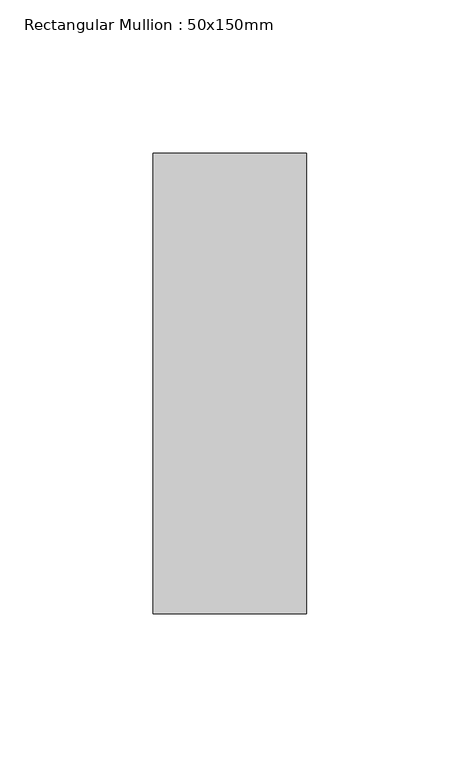
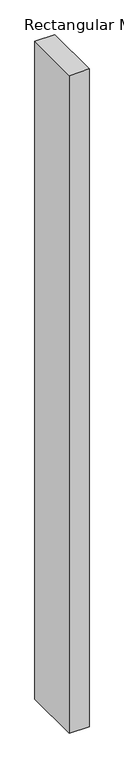
"""IFC4 building model written with IfcOpenShell, lengths in millimetres: member geometry, Rectangular Mullion : 50x150mm."""

from ifc_helpers import new_model, si_unit, frame, origin, place, context, project, spatial, polyline, outline, extrude, source, transform, mapped, element, save


def rectangular_mullion_50x150mm_df7bd136(model_context):
    return source(origin(), model_context, "Body", "SweptSolid", [
        extrude(outline(polyline([(25.0, 75.0), (25.0, -75.0), (-25.0, -75.0), (-25.0, 75.0), (25.0, 75.0)])), frame((0.0, 0.0, -1755.0), z_axis=(0.0, 0.0, 1.0), x_axis=(1.0, 0.0, 0.0)), (0.0, 0.0, 1.0), 1755.0),
    ])


if __name__ == "__main__":
    model = new_model("IFC4")
    model_context = context("Model", 3, world=origin())
    ifc_project = project(units=[si_unit("LENGTHUNIT", "METRE", prefix="MILLI")], contexts=[model_context])
    site = spatial("IfcSite", under=ifc_project)
    building = spatial("IfcBuilding", under=site)
    placement = place(None, origin())
    rectangular_mullion_50x150mm_shape = rectangular_mullion_50x150mm_df7bd136(model_context)
    element("IfcMember", 1, ObjectType="Rectangular Mullion : 50x150mm", at=placement, inside=building, context=model_context, shape_type="MappedRepresentation", body=[
        mapped(rectangular_mullion_50x150mm_shape, transform((0.0, 0.0, 0.0), x_axis=(1.0, 0.0, 0.0), y_axis=(0.0, 1.0, 0.0), z_axis=(0.0, 0.0, 1.0))),
    ])
    save(model, "model.ifc")

# Revit data of these elements
# Type "Rectangular Mullion : 50x150mm"
#   Keynote = "H11"
#   built-in parameter 1007304 = 0.492126 (stored number, unit not read)
#   built-in parameter 1007301 = 0.082021 (stored number, unit not read)
#   built-in parameter 1007300 = 0.082021 (stored number, unit not read)
# Element 1 (IfcMember, "Rectangular Mullion : 50x150mm")
#   Materials on its faces: "Aluminium"
# Materials
#   "Aluminium": class "Metal", colour RGB 247 247 247, transparency 0, Description = "Aluminium 6061", Cost = 0
